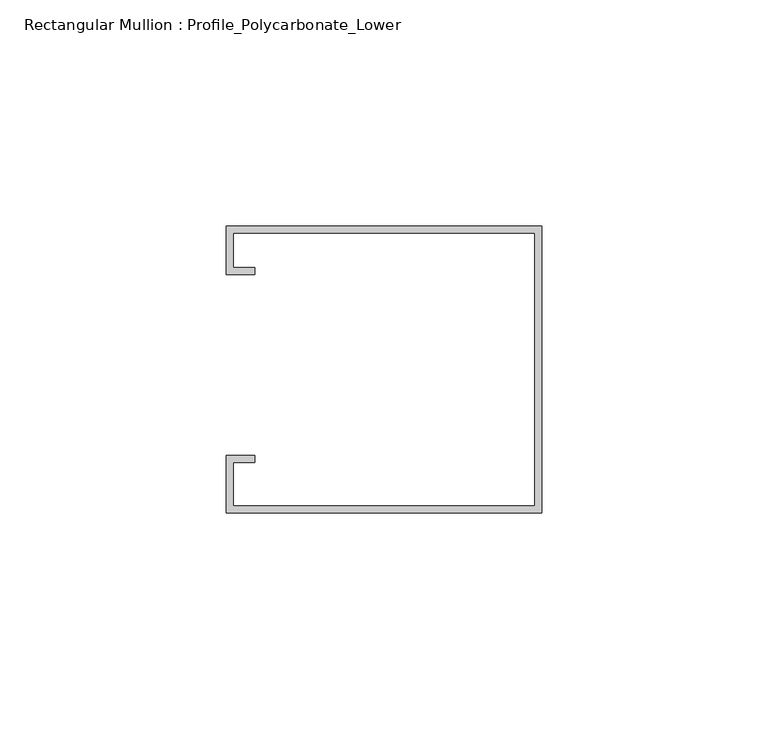
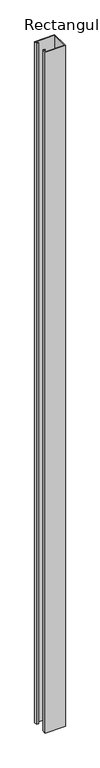
"""IFC4 building model written with IfcOpenShell, lengths in millimetres: member geometry, Rectangular Mullion : Profile_Polycarbonate_Lower."""

import ifcopenshell
import ifcopenshell.guid

model = None  # the IFC model being written
_history = None  # IfcOwnerHistory: only IFC2X3 demands one
_inside = {}  # id of a spatial element -> (the spatial element, [elements in it])
_under = {}  # id of a project, library or spatial element -> (it, [spatial elements below it])
_declared = {}  # id of a project -> (the project, [libraries it declares])
_typed = {}  # id of a type object -> (the type object, [elements of that type])
_made_of = {}  # id of a material, layer set ... -> (it, [elements and type objects made of it])


def new_model(schema):
    """Start an empty IFC model of exactly this schema.

    Asked for "IFC4X3", IfcOpenShell would pick the latest addendum, in which some entities
    have other attributes; the version numbers below select the first issue.
    IFC2X3 requires an IfcOwnerHistory on every rooted entity: one is made here for all.
    """
    global model, _history
    if schema == "IFC4X3":
        model = ifcopenshell.file(schema_version=(4, 3, 0, 0))
    else:
        model = ifcopenshell.file(schema=schema)
    _inside.clear()
    _under.clear()
    _declared.clear()
    _typed.clear()
    _made_of.clear()
    _history = None
    if model.schema == "IFC2X3":
        org = make("IfcOrganization", Name="unknown")
        user = make(
            "IfcPersonAndOrganization",
            ThePerson=make("IfcPerson", FamilyName="unknown"),
            TheOrganization=org,
        )
        app = make(
            "IfcApplication",
            ApplicationDeveloper=org,
            Version="unknown",
            ApplicationFullName="unknown",
            ApplicationIdentifier="unknown",
        )
        _history = make(
            "IfcOwnerHistory",
            OwningUser=user,
            OwningApplication=app,
            ChangeAction="ADDED",
            CreationDate=0,
        )
    return model


def make(cls, **values):
    """One entity of the class cls with the attributes given. An attribute that is None is left unset."""
    return model.create_entity(
        cls, **{name: value for name, value in values.items() if value is not None}
    )


def rooted(cls, **values):
    """An entity with a GlobalId (a new one), such as an element, a storey or a relation."""
    return make(cls, GlobalId=ifcopenshell.guid.new(), OwnerHistory=_history, **values)


def si_unit(unit_type, name, prefix=None):
    """IfcSIUnit, for example si_unit("LENGTHUNIT", "METRE", prefix="MILLI")."""
    return make("IfcSIUnit", UnitType=unit_type, Prefix=prefix, Name=name)


def assignment(units):
    """IfcUnitAssignment: the units of a project."""
    return None if units is None else make("IfcUnitAssignment", Units=units)


def point(xyz):
    """IfcCartesianPoint."""
    return None if xyz is None else make("IfcCartesianPoint", Coordinates=xyz)


def direction(xyz):
    """IfcDirection."""
    return None if xyz is None else make("IfcDirection", DirectionRatios=xyz)


def frame(location, z_axis=None, x_axis=None):
    """IfcAxis2Placement3D, a coordinate frame: its origin and axes. An axis left out is left unset."""
    return make(
        "IfcAxis2Placement3D",
        Location=point(location),
        Axis=direction(z_axis),
        RefDirection=direction(x_axis),
    )


def origin():
    """The frame at (0, 0, 0) with its axes left unset."""
    return frame((0.0, 0.0, 0.0))


def place(relative_to, where):
    """IfcLocalPlacement: puts the frame where relative to a parent placement (None: the world)."""
    return make(
        "IfcLocalPlacement", PlacementRelTo=relative_to, RelativePlacement=where
    )


def context(
    kind, dimensions, precision=None, world=None, true_north=None, identifier=None
):
    """IfcGeometricRepresentationContext, for example the 3D "Model" context."""
    return make(
        "IfcGeometricRepresentationContext",
        ContextIdentifier=identifier,
        ContextType=kind,
        CoordinateSpaceDimension=dimensions,
        Precision=precision,
        WorldCoordinateSystem=world,
        TrueNorth=true_north,
    )


def project(units=None, contexts=None):
    """IfcProject with its units and contexts."""
    return rooted(
        "IfcProject",
        Name="project",
        RepresentationContexts=contexts,
        UnitsInContext=assignment(units),
    )


def spatial(cls, under=None, at=None, **own):
    """A site, building, storey or space (cls), placed at a placement, below another one or the project."""
    s = rooted(cls, ObjectPlacement=at, **own)
    if under is not None:
        _under.setdefault(under.id(), (under, []))[1].append(s)
    return s


def polyline(points):
    """IfcPolyline through the points."""
    return make("IfcPolyline", Points=[point(p) for p in points])


def outline(outer, holes=None, kind="AREA"):
    """IfcArbitraryClosedProfileDef: a profile drawn as a closed curve; with holes, ...WithVoids."""
    if holes is None:
        return make("IfcArbitraryClosedProfileDef", ProfileType=kind, OuterCurve=outer)
    return make(
        "IfcArbitraryProfileDefWithVoids",
        ProfileType=kind,
        OuterCurve=outer,
        InnerCurves=holes,
    )


def extrude(swept, where, along, depth):
    """IfcExtrudedAreaSolid: the profile swept, set in the frame where, extruded along a direction by depth."""
    return make(
        "IfcExtrudedAreaSolid",
        SweptArea=swept,
        Position=where,
        ExtrudedDirection=direction(along),
        Depth=depth,
    )


def shape(context_of_items, identifier, shape_type, items):
    """IfcShapeRepresentation: the items that make up one representation, for example the "Body"."""
    return make(
        "IfcShapeRepresentation",
        ContextOfItems=context_of_items,
        RepresentationIdentifier=identifier,
        RepresentationType=shape_type,
        Items=items,
    )


def source(mapping_origin, context_of_items, identifier, shape_type, items):
    """IfcRepresentationMap: a shape defined once, which mapped items show again and again."""
    return make(
        "IfcRepresentationMap",
        MappingOrigin=mapping_origin,
        MappedRepresentation=shape(context_of_items, identifier, shape_type, items),
    )


def transform(
    local_origin,
    x_axis=None,
    y_axis=None,
    z_axis=None,
    scale=None,
    scale2=None,
    scale3=None,
    uniform=True,
):
    """IfcCartesianTransformationOperator3D, or its non-uniform kind. x_axis, y_axis, z_axis: its Axis1, 2, 3."""
    if uniform:
        return make(
            "IfcCartesianTransformationOperator3D",
            Axis1=direction(x_axis),
            Axis2=direction(y_axis),
            LocalOrigin=point(local_origin),
            Scale=scale,
            Axis3=direction(z_axis),
        )
    return make(
        "IfcCartesianTransformationOperator3DnonUniform",
        Axis1=direction(x_axis),
        Axis2=direction(y_axis),
        LocalOrigin=point(local_origin),
        Scale=scale,
        Axis3=direction(z_axis),
        Scale2=scale2,
        Scale3=scale3,
    )


def mapped(mapping_source, mapping_target):
    """IfcMappedItem: shows the shape of a source again, moved by a transform."""
    return make(
        "IfcMappedItem", MappingSource=mapping_source, MappingTarget=mapping_target
    )


def made_of(thing, what):
    """Note that an element or type object is made of a material, layer set ...; save() writes the relation."""
    if what is not None:
        _made_of.setdefault(what.id(), (what, []))[1].append(thing)
    return thing


def element(
    cls,
    number,
    at=None,
    inside=None,
    cuts=None,
    type_object=None,
    material=None,
    context=None,
    identifier="Body",
    shape_type=None,
    held_by="IfcProductDefinitionShape",
    body=None,
    shapes=None,
    **own,
):
    """One element of the class cls, such as IfcWall. Its Tag is "e" and its number.

    at: its placement. inside: the storey or other place that contains it. cuts: it is an
    opening in that element (IfcRelVoidsElement). A single representation is given by context,
    identifier, shape_type and body (its items); several are given by shapes. held_by: the class
    of the entity that holds the representations. save() writes the other relations.
    """
    e = rooted(cls, Tag="e%d" % number, ObjectPlacement=at, **own)
    if body is not None:
        shapes = [shape(context, identifier, shape_type, body)]
    if shapes is not None:
        e.Representation = make(held_by, Representations=shapes)
    if inside is not None:
        _inside.setdefault(inside.id(), (inside, []))[1].append(e)
    if cuts is not None:
        rooted(
            "IfcRelVoidsElement", RelatingBuildingElement=cuts, RelatedOpeningElement=e
        )
    if type_object is not None:
        _typed.setdefault(type_object.id(), (type_object, []))[1].append(e)
    return made_of(e, material)


def aggregate(whole, parts):
    """IfcRelAggregates: a whole, such as a stair, and the parts it consists of."""
    return rooted("IfcRelAggregates", RelatingObject=whole, RelatedObjects=parts)


def save(model, path):
    """Write the relations noted so far, then the file.

    IfcRelAggregates (storeys below a building ...), IfcRelContainedInSpatialStructure (elements
    in a storey), IfcRelDefinesByType, IfcRelAssociatesMaterial and IfcRelDeclares: one each for
    every whole, place, type object, material and project.
    """
    for whole, parts in _under.values():
        aggregate(whole, parts)
    for where, things in _inside.values():
        rooted(
            "IfcRelContainedInSpatialStructure",
            RelatedElements=things,
            RelatingStructure=where,
        )
    for kind, things in _typed.values():
        rooted("IfcRelDefinesByType", RelatedObjects=things, RelatingType=kind)
    for what, things in _made_of.values():
        rooted("IfcRelAssociatesMaterial", RelatedObjects=things, RelatingMaterial=what)
    for by, libraries in _declared.values():
        rooted("IfcRelDeclares", RelatingContext=by, RelatedDefinitions=libraries)
    model.write(path)


def rectangular_mullion_profile_polycarbonate_lower_0f329726(model_context):
    return source(origin(), model_context, "Body", "SweptSolid", [
        extrude(outline(polyline([(0.0, -32.7), (-69.85, -32.7), (-69.85, -20.0), (-63.5, -20.0), (-63.5, -21.5875), (-68.2625, -21.5875), (-68.2625, -31.1125), (-1.5875, -31.1125), (-1.5875, 29.2125), (-68.2625, 29.2125), (-68.2625, 21.5875), (-63.5, 21.5875), (-63.5, 20.0), (-69.85, 20.0), (-69.85, 30.8), (0.0, 30.8), (0.0, -32.7)])), frame((0.0, 0.0, -2505.075), z_axis=(0.0, 0.0, 1.0), x_axis=(1.0, 0.0, 0.0)), (0.0, 0.0, 1.0), 2505.075),
    ])


if __name__ == "__main__":
    model = new_model("IFC4")
    model_context = context("Model", 3, world=origin())
    ifc_project = project(units=[si_unit("LENGTHUNIT", "METRE", prefix="MILLI")], contexts=[model_context])
    site = spatial("IfcSite", under=ifc_project)
    building = spatial("IfcBuilding", under=site)
    placement = place(None, origin())
    rectangular_mullion_profile_polycarbonate_lower_shape = rectangular_mullion_profile_polycarbonate_lower_0f329726(model_context)
    element("IfcMember", 1, ObjectType="Rectangular Mullion : Profile_Polycarbonate_Lower", at=placement, inside=building, context=model_context, shape_type="MappedRepresentation", body=[
        mapped(rectangular_mullion_profile_polycarbonate_lower_shape, transform((0.0, 0.0, 0.0), x_axis=(1.0, 0.0, 0.0), y_axis=(0.0, 1.0, 0.0), z_axis=(0.0, 0.0, 1.0))),
    ])
    save(model, "model.ifc")

# Revit data of these elements
# Type "Rectangular Mullion : Profile_Polycarbonate_Lower"
#   built-in parameter 1007322 = 0.208333 (stored number, unit not read)
#   built-in parameter 1007321 = 0 (stored number, unit not read)
#   built-in parameter 1007320 = 0.00520833 (stored number, unit not read)
# Element 1 (IfcMember, "Rectangular Mullion : Profile_Polycarbonate_Lower")
#   Materials on its faces: "ALUMINUM PROFILE AT POLYCARBONATE PANEL"
# Materials
#   "ALUMINUM PROFILE AT POLYCARBONATE PANEL": class "Metal", colour RGB 244 244 244, transparency 0, Description = "Aluminum 6061", Cost = 0
